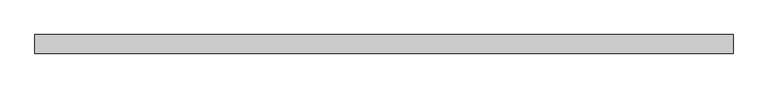
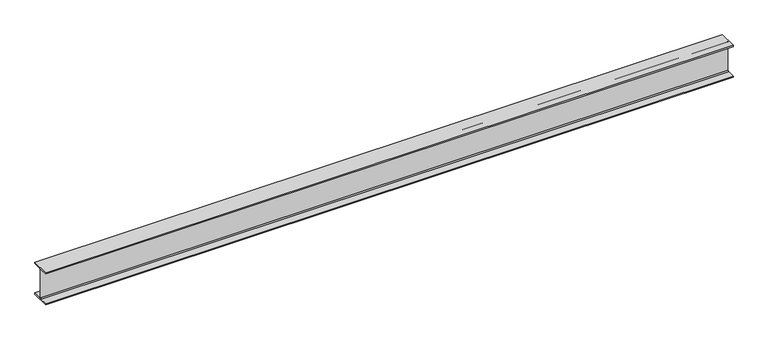
"""IFC4 building model written with IfcOpenShell, lengths in millimetres: beam geometry, Old_Steel Beam_H-KSD3502 : H_SB_ASB_H-340×250x9x14."""

from ifc_helpers import new_model, si_unit, point, frame, frame_2d, origin, place, context, project, spatial, polyline, circle_curve, trimmed, segment, composite_curve, outline, extrude, source, transform, mapped, element, save


def beam_69bffec9(model_context):
    return source(origin(), model_context, "Body", "SweptSolid", [
        extrude(outline(composite_curve([segment(polyline([(82.5, -141.5), (82.5, -151.7), (-82.5, -151.7), (-82.5, -141.5), (-11.9, -141.5)]), True, "CONTINUOUS"), segment(trimmed(circle_curve(frame_2d((-11.9, -132.6)), 8.9), [point((-11.9, -141.5))], [point((-3.0, -132.6))], True, "CARTESIAN"), True, "CONTINUOUS"), segment(polyline([(-3.0, -132.6), (-3.0, 132.6)]), True, "CONTINUOUS"), segment(trimmed(circle_curve(frame_2d((-11.9, 132.6)), 8.9), [point((-3.0, 132.6))], [point((-11.9, 141.5))], True, "CARTESIAN"), True, "CONTINUOUS"), segment(polyline([(-11.9, 141.5), (-82.5, 141.5), (-82.5, 151.7), (82.5, 151.7), (82.5, 141.5), (11.9, 141.5)]), True, "CONTINUOUS"), segment(trimmed(circle_curve(frame_2d((11.9, 132.6)), 8.9), [point((11.9, 141.5))], [point((3.0, 132.6))], True, "CARTESIAN"), True, "CONTINUOUS"), segment(polyline([(3.0, 132.6), (3.0, -132.6)]), True, "CONTINUOUS"), segment(trimmed(circle_curve(frame_2d((11.9, -132.6)), 8.9), [point((3.0, -132.6))], [point((11.9, -141.5))], True, "CARTESIAN"), True, "CONTINUOUS"), segment(polyline([(11.9, -141.5), (82.5, -141.5)]), True, "CONTINUOUS")], self_intersect=False)), frame((-3087.3, 0.0, 0.0), z_axis=(1.0, 0.0, 0.0), x_axis=(0.0, 1.0, 0.0)), (0.0, 0.0, 1.0), 6174.6),
    ])


if __name__ == "__main__":
    model = new_model("IFC4")
    model_context = context("Model", 3, world=origin())
    ifc_project = project(units=[si_unit("LENGTHUNIT", "METRE", prefix="MILLI")], contexts=[model_context])
    site = spatial("IfcSite", under=ifc_project)
    building = spatial("IfcBuilding", under=site)
    placement = place(None, origin())
    beam_shape = beam_69bffec9(model_context)
    element("IfcBeam", 1, ObjectType="Old_Steel Beam_H-KSD3502 : H_SB_ASB_H-340×250x9x14", at=placement, inside=building, context=model_context, shape_type="MappedRepresentation", body=[
        mapped(beam_shape, transform((0.0, 0.0, 0.0), x_axis=(1.0, 0.0, 0.0), y_axis=(0.0, 1.0, 0.0), z_axis=(0.0, 0.0, 1.0))),
    ])
    save(model, "model.ifc")

# Revit data of these elements
# Type "Old_Steel Beam_H-KSD3502 : H_SB_ASB_H-340×250x9x14"
#   Width = 25.0 cm
#   Web Thickness = 0.9 cm
#   Web Fillet = 2.0 cm
#   Warping Constant = 968661.0 cm⁶
#   Torsional Moment of Inertia = 53.6551 cm⁴
#   Torsional Modulus = 1.0 cm³
#   Section Area = 101.5 cm²
#   Plastic Modulus weak axis = 447.0 cm³
#   Plastic Modulus strong axis = 1410.0 cm³
#   Perimeter = 1.63 m²/m
#   Nominal Weight = 79.70 kgf/m
#   Moment of Inertia weak axis = 3650.00 cm⁴
#   Moment of Inertia strong axis = 21700.00 cm⁴
#   Height = 34.0 cm
#   Flange Thickness = 1.4 cm
#   Elastic Modulus weak axis = 292.0 cm³
#   Elastic Modulus strong axis = 1280.0 cm³
#   Centroid Vertical = 17.0 cm
#   Centroid Horizontal = 12.5 cm
#   Length [instance default] = 1.5240 m
#   Structural Material [instance default] = Steel, 45-345
#   Assembly Code = ""
# Element 1 (IfcBeam, "Old_Steel Beam_H-KSD3502 : H_SB_ASB_H-340×250x9x14")
#   Structural Material = none
# Materials
#   "Steel, 45-345": class "Metal", colour RGB 189 187 185, transparency 0, Description = "Steel 345 MPa", Cost = 0
